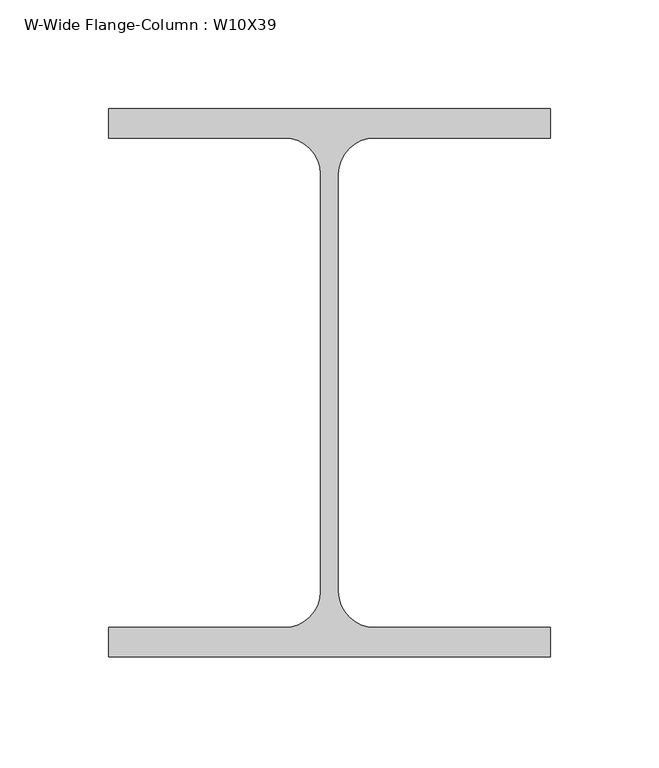
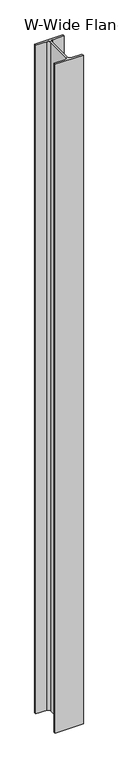
"""IFC4 building model written with IfcOpenShell, lengths in millimetres: column geometry, W-Wide Flange-Column : W10X39."""

from ifc_helpers import new_model, si_unit, point, frame, frame_2d, origin, place, context, project, spatial, polyline, circle_curve, trimmed, segment, composite_curve, outline, extrude, source, transform, mapped, element, save


def w_wide_flange_column_w10x39_652f0938(model_context):
    return source(origin(), model_context, "Body", "SweptSolid", [
        extrude(outline(composite_curve([segment(polyline([(101.473, 125.984), (101.473, 112.522), (20.701, 112.522)]), True, "CONTINUOUS"), segment(trimmed(circle_curve(frame_2d((20.701, 95.8215)), 16.7005), [point((20.701, 112.522))], [point((4.0005, 95.8215))], True, "CARTESIAN"), True, "CONTINUOUS"), segment(polyline([(4.0005, 95.8215), (4.0005, -95.8215)]), True, "CONTINUOUS"), segment(trimmed(circle_curve(frame_2d((20.701, -95.8215)), 16.7005), [point((4.0005, -95.8215))], [point((20.701, -112.522))], True, "CARTESIAN"), True, "CONTINUOUS"), segment(polyline([(20.701, -112.522), (101.473, -112.522), (101.473, -125.984), (-101.473, -125.984), (-101.473, -112.522), (-20.701, -112.522)]), True, "CONTINUOUS"), segment(trimmed(circle_curve(frame_2d((-20.701, -95.8215)), 16.7005), [point((-20.701, -112.522))], [point((-4.0005, -95.8215))], True, "CARTESIAN"), True, "CONTINUOUS"), segment(polyline([(-4.0005, -95.8215), (-4.0005, 95.8215)]), True, "CONTINUOUS"), segment(trimmed(circle_curve(frame_2d((-20.701, 95.8215)), 16.7005), [point((-4.0005, 95.8215))], [point((-20.701, 112.522))], True, "CARTESIAN"), True, "CONTINUOUS"), segment(polyline([(-20.701, 112.522), (-101.473, 112.522), (-101.473, 125.984), (101.473, 125.984)]), True, "CONTINUOUS")], self_intersect=False)), frame((0.0, 0.0, 12566.65), z_axis=(0.0, 0.0, 1.0), x_axis=(1.0, 0.0, 0.0)), (0.0, 0.0, 1.0), 5060.95),
    ])


if __name__ == "__main__":
    model = new_model("IFC4")
    model_context = context("Model", 3, world=origin())
    ifc_project = project(units=[si_unit("LENGTHUNIT", "METRE", prefix="MILLI")], contexts=[model_context])
    site = spatial("IfcSite", under=ifc_project)
    building = spatial("IfcBuilding", under=site)
    placement = place(None, origin())
    w_wide_flange_column_w10x39_shape = w_wide_flange_column_w10x39_652f0938(model_context)
    element("IfcColumn", 1, ObjectType="W-Wide Flange-Column : W10X39", at=placement, inside=building, context=model_context, shape_type="MappedRepresentation", body=[
        mapped(w_wide_flange_column_w10x39_shape, transform((0.0, 0.0, 0.0), x_axis=(1.0, 0.0, 0.0), y_axis=(0.0, 1.0, 0.0), z_axis=(0.0, 0.0, 1.0))),
    ])
    save(model, "model.ifc")

# Revit data of these elements
# Type "W-Wide Flange-Column : W10X39"
#   Assembly Code = "B10"
#   W = 39
#   bf = 0' - 7.99"
#   d = 0' - 9.92"
#   k = 0' - 1 3/16"
#   kr = 0' - 0.6575"
#   tf = 0' - 0.53"
#   tw = 0' - 0.315"
#   A = 0.0798611 SF
#   Structural Material [instance default] = Steel ASTM A992
# Element 1 (IfcColumn, "W-Wide Flange-Column : W10X39")
#   Materials on its faces: "Steel ASTM A992"
# Materials
#   "Steel ASTM A992": class "Metal", colour RGB 199 199 199, transparency 0, Description = "Structural steel 50ksi", Cost = 0
